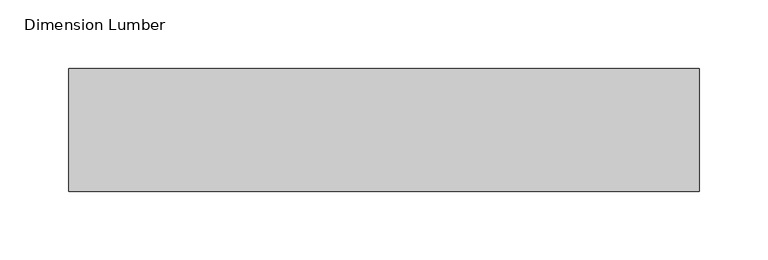
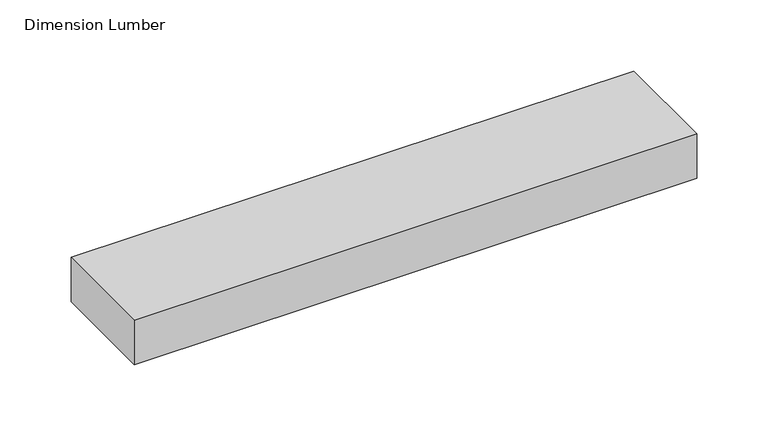
"""IFC4 building model written with IfcOpenShell, lengths in millimetres: beam geometry, Dimension Lumber : Top Supporting Lumbers."""

from ifc_helpers import new_model, si_unit, frame, origin, place, context, project, spatial, polyline, outline, extrude, source, transform, mapped, element, save


def dimension_lumber_f425b765(model_context):
    return source(origin(), model_context, "Body", "SweptSolid", [
        extrude(outline(polyline([(292.0, 44.45), (292.0, -44.45), (-165.0, -44.45), (-165.0, 44.45), (292.0, 44.45)])), frame((0.0, 0.0, -19.05), z_axis=(0.0, 0.0, 1.0), x_axis=(1.0, 0.0, 0.0)), (0.0, 0.0, 1.0), 38.1),
    ])


if __name__ == "__main__":
    model = new_model("IFC4")
    model_context = context("Model", 3, world=origin())
    ifc_project = project(units=[si_unit("LENGTHUNIT", "METRE", prefix="MILLI")], contexts=[model_context])
    site = spatial("IfcSite", under=ifc_project)
    building = spatial("IfcBuilding", under=site)
    placement = place(None, origin())
    dimension_lumber_shape = dimension_lumber_f425b765(model_context)
    element("IfcBeam", 1, ObjectType="Dimension Lumber : Top Supporting Lumbers", at=placement, inside=building, context=model_context, shape_type="MappedRepresentation", body=[
        mapped(dimension_lumber_shape, transform((0.0, 0.0, 0.0), x_axis=(1.0, 0.0, 0.0), y_axis=(0.0, 1.0, 0.0), z_axis=(0.0, 0.0, 1.0))),
    ])
    save(model, "model.ifc")

# Revit data of these elements
# Type "Dimension Lumber : Top Supporting Lumbers"
#   Assembly Code = "B10"
#   A = 0.0364583 SF
#   Length [instance default] = 5' - 0"
#   b = 0' - 3 1/2"
#   d = 0' - 1 1/2"
#   Structural Material [instance default] = Softwood, Lumber
# Element 1 (IfcBeam, "Dimension Lumber : Top Supporting Lumbers")
#   Structural Material = Douglas Fir #2
#   Materials on its faces: "Douglas Fir #2"
# Materials
#   "Softwood, Lumber": class "Wood", colour RGB 223 192 134, transparency 0, Description = "Pinus Echinata", Cost = 0
#   "Douglas Fir #2": class "Wood", colour RGB 223 192 134, transparency 0, Description = "Pinus Echinata", Cost = 0
